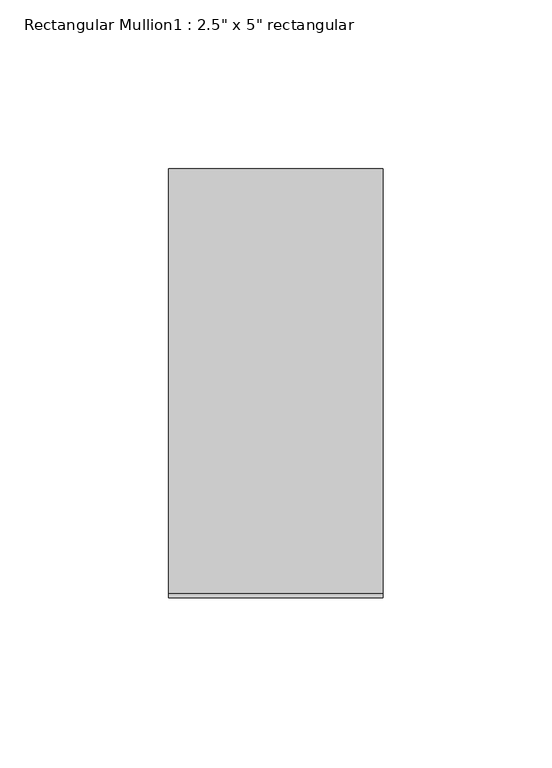
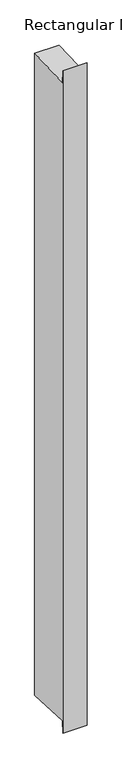
"""IFC4 building model written with IfcOpenShell, lengths in millimetres: member geometry."""

from ifc_helpers import new_model, si_unit, frame, origin, place, context, project, spatial, polyline, outline, extrude, source, transform, mapped, element, save


def member_7b0b344d(model_context):
    return source(origin(), model_context, "Body", "SweptSolid", [
        extrude(outline(polyline([(-63.5, 30.4748075), (-62.174126, -2.5237591), (63.5, 2.5257955), (63.5, -1767.8257955), (-62.174126, -1762.7762409), (-63.5, -1795.7748075), (-63.5, 30.4748075)])), frame((-63.5, 0.0, 0.0), z_axis=(1.0, 0.0, 0.0), x_axis=(0.0, 1.0, 0.0)), (0.0, 0.0, 1.0), 63.5),
    ])


if __name__ == "__main__":
    model = new_model("IFC4")
    model_context = context("Model", 3, world=origin())
    ifc_project = project(units=[si_unit("LENGTHUNIT", "METRE", prefix="MILLI")], contexts=[model_context])
    site = spatial("IfcSite", under=ifc_project)
    building = spatial("IfcBuilding", under=site)
    placement = place(None, origin())
    member_shape = member_7b0b344d(model_context)
    element("IfcMember", 1, ObjectType="Rectangular Mullion1 : 2.5\" x 5\" rectangular", at=placement, inside=building, context=model_context, shape_type="MappedRepresentation", body=[
        mapped(member_shape, transform((0.0, 0.0, 0.0), x_axis=(1.0, 0.0, 0.0), y_axis=(0.0, 1.0, 0.0), z_axis=(0.0, 0.0, 1.0))),
    ])
    save(model, "model.ifc")

# Revit data of these elements
# Type "Rectangular Mullion1 : 2.5\" x 5\" rectangular"
#   built-in parameter 1007304 = 0.416667 (stored number, unit not read)
#   built-in parameter 1007301 = 0.104167 (stored number, unit not read)
#   built-in parameter 1007300 = 0.104167 (stored number, unit not read)
# Element 1 (IfcMember, "Rectangular Mullion1 : 2.5\" x 5\" rectangular")
#   Materials on its faces: "support-frame"
# Materials
#   "support-frame": class "Unassigned", colour RGB 233 233 233, transparency 0, Cost = 0
